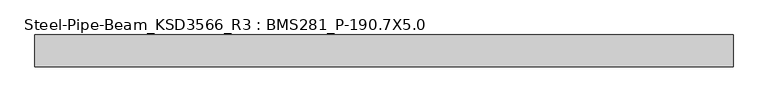
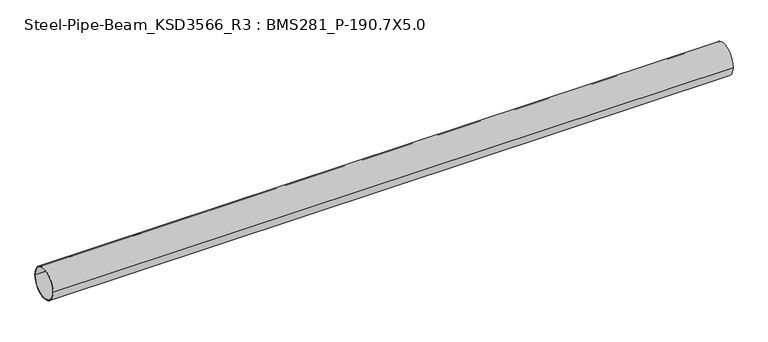
"""IFC4 building model written with IfcOpenShell, lengths in millimetres: member geometry, Steel-Pipe-Beam_KSD3566_R3 : BMS281_P-190.7X5.0."""

from ifc_helpers import new_model, si_unit, point, frame, origin, origin_2d, place, context, project, spatial, circle_curve, trimmed, segment, composite_curve, outline, extrude, source, transform, mapped, element, save


def steel_pipe_beam_ksd3566_r3_bms281_p_190_7x5_0_0cb403fb(model_context):
    return source(origin(), model_context, "Body", "SweptSolid", [
        extrude(outline(composite_curve([segment(trimmed(circle_curve(origin_2d(), 95.35), [point((-95.35, 0.0))], [point((95.35, 0.0))], False, "CARTESIAN"), True, "CONTINUOUS"), segment(trimmed(circle_curve(origin_2d(), 95.35), [point((95.35, 0.0))], [point((-95.35, 0.0))], False, "CARTESIAN"), True, "CONTINUOUS")], self_intersect=False), holes=[composite_curve([segment(trimmed(circle_curve(origin_2d(), 90.35), [point((90.35, 0.0))], [point((-90.35, 0.0))], True, "CARTESIAN"), True, "CONTINUOUS"), segment(trimmed(circle_curve(origin_2d(), 90.35), [point((-90.35, 0.0))], [point((90.35, 0.0))], True, "CARTESIAN"), True, "CONTINUOUS")], self_intersect=False)]), frame((-2093.8610652, 0.0, 0.0), z_axis=(1.0, 0.0, 0.0), x_axis=(0.0, 1.0, 0.0)), (0.0, 0.0, 1.0), 4153.366687),
    ])


if __name__ == "__main__":
    model = new_model("IFC4")
    model_context = context("Model", 3, world=origin())
    ifc_project = project(units=[si_unit("LENGTHUNIT", "METRE", prefix="MILLI")], contexts=[model_context])
    site = spatial("IfcSite", under=ifc_project)
    building = spatial("IfcBuilding", under=site)
    placement = place(None, origin())
    steel_pipe_beam_ksd3566_r3_bms281_p_190_7x5_0_shape = steel_pipe_beam_ksd3566_r3_bms281_p_190_7x5_0_0cb403fb(model_context)
    element("IfcMember", 1, ObjectType="Steel-Pipe-Beam_KSD3566_R3 : BMS281_P-190.7X5.0", at=placement, inside=building, context=model_context, shape_type="MappedRepresentation", body=[
        mapped(steel_pipe_beam_ksd3566_r3_bms281_p_190_7x5_0_shape, transform((0.0, 0.0, 0.0), x_axis=(1.0, 0.0, 0.0), y_axis=(0.0, 1.0, 0.0), z_axis=(0.0, 0.0, 1.0))),
    ])
    save(model, "model.ifc")

# Revit data of these elements
# Type "Steel-Pipe-Beam_KSD3566_R3 : BMS281_P-190.7X5.0"
#   Keynote = "P-190.7X5.0"
#   SteelWeight = "Light"
#   t = 0.0050 m
#   Surface Area = 0.599102 m²/m
#   Section Area = 29.1697 cm²
#   Mass per Unit Length = 22.8982 kg/m
#   Length [instance default] = 1.5000 m
#   D = 0.1907 m
#   hec_material4 [instance default] = none
#   hec_material3 [instance default] = none
#   hec_material2 [instance default] = none
#   hec_material1 [instance default] = none
#   Structural Material [instance default] = Steel, 45-345
#   Assembly Code = ""
# Element 1 (IfcMember, "Steel-Pipe-Beam_KSD3566_R3 : BMS281_P-190.7X5.0")
#   Structural Material = none
# Materials
#   "Steel, 45-345": class "Metal", colour RGB 189 187 185, transparency 0, Description = "Steel 345 MPa", Cost = 0
